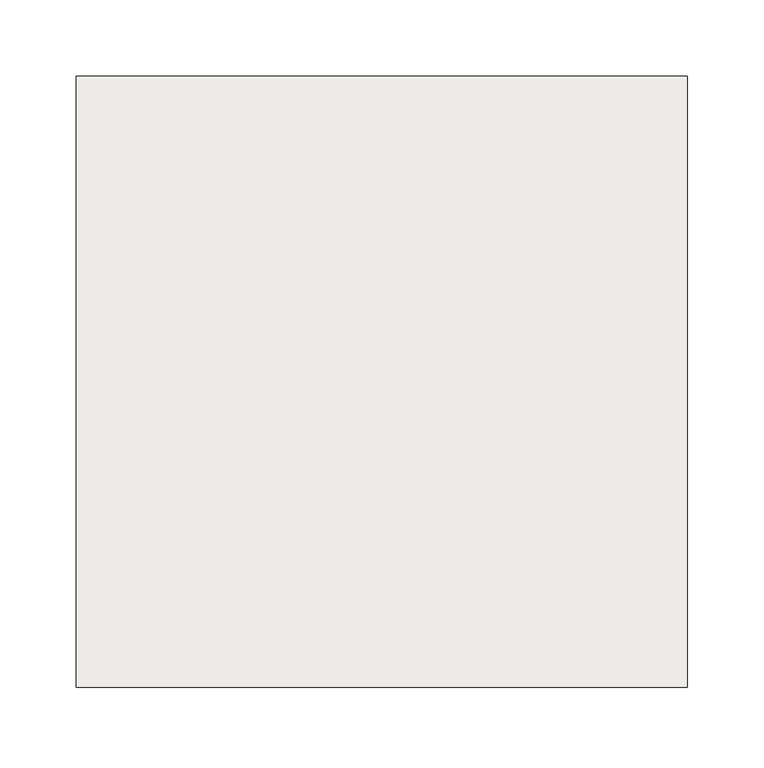
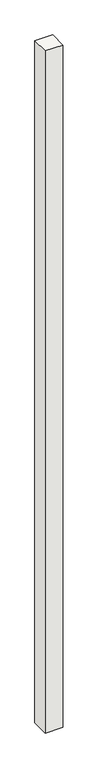
"""IFC4 building model written with IfcOpenShell, lengths in millimetres: footing geometry, NLRS_17_SFO_TLB_funderingspaal geheid beton prefab-AV-MMBPC_gen_rsf : heipaal beton prefab_gen__bxh 400x400."""

import ifcopenshell
import ifcopenshell.guid

model = None  # the IFC model being written
_history = None  # IfcOwnerHistory: only IFC2X3 demands one
_inside = {}  # id of a spatial element -> (the spatial element, [elements in it])
_under = {}  # id of a project, library or spatial element -> (it, [spatial elements below it])
_declared = {}  # id of a project -> (the project, [libraries it declares])
_typed = {}  # id of a type object -> (the type object, [elements of that type])
_made_of = {}  # id of a material, layer set ... -> (it, [elements and type objects made of it])


def new_model(schema):
    """Start an empty IFC model of exactly this schema.

    Asked for "IFC4X3", IfcOpenShell would pick the latest addendum, in which some entities
    have other attributes; the version numbers below select the first issue.
    IFC2X3 requires an IfcOwnerHistory on every rooted entity: one is made here for all.
    """
    global model, _history
    if schema == "IFC4X3":
        model = ifcopenshell.file(schema_version=(4, 3, 0, 0))
    else:
        model = ifcopenshell.file(schema=schema)
    _inside.clear()
    _under.clear()
    _declared.clear()
    _typed.clear()
    _made_of.clear()
    _history = None
    if model.schema == "IFC2X3":
        org = make("IfcOrganization", Name="unknown")
        user = make(
            "IfcPersonAndOrganization",
            ThePerson=make("IfcPerson", FamilyName="unknown"),
            TheOrganization=org,
        )
        app = make(
            "IfcApplication",
            ApplicationDeveloper=org,
            Version="unknown",
            ApplicationFullName="unknown",
            ApplicationIdentifier="unknown",
        )
        _history = make(
            "IfcOwnerHistory",
            OwningUser=user,
            OwningApplication=app,
            ChangeAction="ADDED",
            CreationDate=0,
        )
    return model


def make(cls, **values):
    """One entity of the class cls with the attributes given. An attribute that is None is left unset."""
    return model.create_entity(
        cls, **{name: value for name, value in values.items() if value is not None}
    )


def rooted(cls, **values):
    """An entity with a GlobalId (a new one), such as an element, a storey or a relation."""
    return make(cls, GlobalId=ifcopenshell.guid.new(), OwnerHistory=_history, **values)


def si_unit(unit_type, name, prefix=None):
    """IfcSIUnit, for example si_unit("LENGTHUNIT", "METRE", prefix="MILLI")."""
    return make("IfcSIUnit", UnitType=unit_type, Prefix=prefix, Name=name)


def assignment(units):
    """IfcUnitAssignment: the units of a project."""
    return None if units is None else make("IfcUnitAssignment", Units=units)


def point(xyz):
    """IfcCartesianPoint."""
    return None if xyz is None else make("IfcCartesianPoint", Coordinates=xyz)


def direction(xyz):
    """IfcDirection."""
    return None if xyz is None else make("IfcDirection", DirectionRatios=xyz)


def frame(location, z_axis=None, x_axis=None):
    """IfcAxis2Placement3D, a coordinate frame: its origin and axes. An axis left out is left unset."""
    return make(
        "IfcAxis2Placement3D",
        Location=point(location),
        Axis=direction(z_axis),
        RefDirection=direction(x_axis),
    )


def origin():
    """The frame at (0, 0, 0) with its axes left unset."""
    return frame((0.0, 0.0, 0.0))


def place(relative_to, where):
    """IfcLocalPlacement: puts the frame where relative to a parent placement (None: the world)."""
    return make(
        "IfcLocalPlacement", PlacementRelTo=relative_to, RelativePlacement=where
    )


def context(
    kind, dimensions, precision=None, world=None, true_north=None, identifier=None
):
    """IfcGeometricRepresentationContext, for example the 3D "Model" context."""
    return make(
        "IfcGeometricRepresentationContext",
        ContextIdentifier=identifier,
        ContextType=kind,
        CoordinateSpaceDimension=dimensions,
        Precision=precision,
        WorldCoordinateSystem=world,
        TrueNorth=true_north,
    )


def project(units=None, contexts=None):
    """IfcProject with its units and contexts."""
    return rooted(
        "IfcProject",
        Name="project",
        RepresentationContexts=contexts,
        UnitsInContext=assignment(units),
    )


def spatial(cls, under=None, at=None, **own):
    """A site, building, storey or space (cls), placed at a placement, below another one or the project."""
    s = rooted(cls, ObjectPlacement=at, **own)
    if under is not None:
        _under.setdefault(under.id(), (under, []))[1].append(s)
    return s


def polyline(points):
    """IfcPolyline through the points."""
    return make("IfcPolyline", Points=[point(p) for p in points])


def outline(outer, holes=None, kind="AREA"):
    """IfcArbitraryClosedProfileDef: a profile drawn as a closed curve; with holes, ...WithVoids."""
    if holes is None:
        return make("IfcArbitraryClosedProfileDef", ProfileType=kind, OuterCurve=outer)
    return make(
        "IfcArbitraryProfileDefWithVoids",
        ProfileType=kind,
        OuterCurve=outer,
        InnerCurves=holes,
    )


def extrude(swept, where, along, depth):
    """IfcExtrudedAreaSolid: the profile swept, set in the frame where, extruded along a direction by depth."""
    return make(
        "IfcExtrudedAreaSolid",
        SweptArea=swept,
        Position=where,
        ExtrudedDirection=direction(along),
        Depth=depth,
    )


def shape(context_of_items, identifier, shape_type, items):
    """IfcShapeRepresentation: the items that make up one representation, for example the "Body"."""
    return make(
        "IfcShapeRepresentation",
        ContextOfItems=context_of_items,
        RepresentationIdentifier=identifier,
        RepresentationType=shape_type,
        Items=items,
    )


def source(mapping_origin, context_of_items, identifier, shape_type, items):
    """IfcRepresentationMap: a shape defined once, which mapped items show again and again."""
    return make(
        "IfcRepresentationMap",
        MappingOrigin=mapping_origin,
        MappedRepresentation=shape(context_of_items, identifier, shape_type, items),
    )


def transform(
    local_origin,
    x_axis=None,
    y_axis=None,
    z_axis=None,
    scale=None,
    scale2=None,
    scale3=None,
    uniform=True,
):
    """IfcCartesianTransformationOperator3D, or its non-uniform kind. x_axis, y_axis, z_axis: its Axis1, 2, 3."""
    if uniform:
        return make(
            "IfcCartesianTransformationOperator3D",
            Axis1=direction(x_axis),
            Axis2=direction(y_axis),
            LocalOrigin=point(local_origin),
            Scale=scale,
            Axis3=direction(z_axis),
        )
    return make(
        "IfcCartesianTransformationOperator3DnonUniform",
        Axis1=direction(x_axis),
        Axis2=direction(y_axis),
        LocalOrigin=point(local_origin),
        Scale=scale,
        Axis3=direction(z_axis),
        Scale2=scale2,
        Scale3=scale3,
    )


def mapped(mapping_source, mapping_target):
    """IfcMappedItem: shows the shape of a source again, moved by a transform."""
    return make(
        "IfcMappedItem", MappingSource=mapping_source, MappingTarget=mapping_target
    )


def made_of(thing, what):
    """Note that an element or type object is made of a material, layer set ...; save() writes the relation."""
    if what is not None:
        _made_of.setdefault(what.id(), (what, []))[1].append(thing)
    return thing


def element(
    cls,
    number,
    at=None,
    inside=None,
    cuts=None,
    type_object=None,
    material=None,
    context=None,
    identifier="Body",
    shape_type=None,
    held_by="IfcProductDefinitionShape",
    body=None,
    shapes=None,
    **own,
):
    """One element of the class cls, such as IfcWall. Its Tag is "e" and its number.

    at: its placement. inside: the storey or other place that contains it. cuts: it is an
    opening in that element (IfcRelVoidsElement). A single representation is given by context,
    identifier, shape_type and body (its items); several are given by shapes. held_by: the class
    of the entity that holds the representations. save() writes the other relations.
    """
    e = rooted(cls, Tag="e%d" % number, ObjectPlacement=at, **own)
    if body is not None:
        shapes = [shape(context, identifier, shape_type, body)]
    if shapes is not None:
        e.Representation = make(held_by, Representations=shapes)
    if inside is not None:
        _inside.setdefault(inside.id(), (inside, []))[1].append(e)
    if cuts is not None:
        rooted(
            "IfcRelVoidsElement", RelatingBuildingElement=cuts, RelatedOpeningElement=e
        )
    if type_object is not None:
        _typed.setdefault(type_object.id(), (type_object, []))[1].append(e)
    return made_of(e, material)


def aggregate(whole, parts):
    """IfcRelAggregates: a whole, such as a stair, and the parts it consists of."""
    return rooted("IfcRelAggregates", RelatingObject=whole, RelatedObjects=parts)


def save(model, path):
    """Write the relations noted so far, then the file.

    IfcRelAggregates (storeys below a building ...), IfcRelContainedInSpatialStructure (elements
    in a storey), IfcRelDefinesByType, IfcRelAssociatesMaterial and IfcRelDeclares: one each for
    every whole, place, type object, material and project.
    """
    for whole, parts in _under.values():
        aggregate(whole, parts)
    for where, things in _inside.values():
        rooted(
            "IfcRelContainedInSpatialStructure",
            RelatedElements=things,
            RelatingStructure=where,
        )
    for kind, things in _typed.values():
        rooted("IfcRelDefinesByType", RelatedObjects=things, RelatingType=kind)
    for what, things in _made_of.values():
        rooted("IfcRelAssociatesMaterial", RelatedObjects=things, RelatingMaterial=what)
    for by, libraries in _declared.values():
        rooted("IfcRelDeclares", RelatingContext=by, RelatedDefinitions=libraries)
    model.write(path)


def footing_98706cf3(model_context):
    return source(origin(), model_context, "Body", "SweptSolid", [
        extrude(outline(polyline([(200.0, -200.0), (-200.0, -200.0), (-200.0, 200.0), (200.0, 200.0), (200.0, -200.0)])), frame((0.0, 0.0, -20000.0), z_axis=(0.0, 0.0, 1.0), x_axis=(1.0, 0.0, 0.0)), (0.0, 0.0, 1.0), 16280.0),
    ])


if __name__ == "__main__":
    model = new_model("IFC4")
    model_context = context("Model", 3, world=origin())
    ifc_project = project(units=[si_unit("LENGTHUNIT", "METRE", prefix="MILLI")], contexts=[model_context])
    site = spatial("IfcSite", under=ifc_project)
    building = spatial("IfcBuilding", under=site)
    placement = place(None, origin())
    footing_shape = footing_98706cf3(model_context)
    element("IfcFooting", 1, ObjectType="NLRS_17_SFO_TLB_funderingspaal geheid beton prefab-AV-MMBPC_gen_rsf : heipaal beton prefab_gen__bxh 400x400", at=placement, inside=building, context=model_context, shape_type="MappedRepresentation", body=[
        mapped(footing_shape, transform((0.0, 0.0, 0.0), x_axis=(1.0, 0.0, 0.0), y_axis=(0.0, 1.0, 0.0), z_axis=(0.0, 0.0, 1.0))),
    ])
    save(model, "model.ifc")

# Revit data of these elements
# Type "NLRS_17_SFO_TLB_funderingspaal geheid beton prefab-AV-MMBPC_gen_rsf : heipaal beton prefab_gen__bxh 400x400"
#   IfcExportAs = "IfcPile"
#   Type Comments = "prefab heipaal 400x400"
#   Model = " "
#   Manufacturer = " "
#   Description = "prefab heipaal 400x400"
#   Assembly Code = "17.21"
#   Width = 400 mm
#   Slanted Angle [instance default] = 0.00°
#   NLRS_S_draagvermogen_trek [instance default] = 0.00 kN
#   NLRS_S_draagvermogen_druk [instance default] = 0.00 kN
#   NLRS_C_lengte [instance default] = 1660 mm
#   NLRS_C_hoogte = 400 mm
#   NLRS_C_breedte = 400 mm
#   Height [instance default] = 1660 mm
#   Length [instance default] = 1660 mm
#   Angle [instance default] = 0.00°
#   Slanted [instance default] = 0
#   Structural Material = NLRS_f2_beton prefab_gen_rsf
#   Keynote = ""
# Element 1 (IfcFooting, "NLRS_17_SFO_TLB_funderingspaal geheid beton prefab-AV-MMBPC_gen_rsf : heipaal beton prefab_gen__bxh 400x400")
#   NLRS_C_lengte = 16280 mm
#   Height = 16280 mm
#   Length = 16280 mm
#   Materials on its faces: "NLRS_f2_beton prefab_gen_rsf"
# Materials
#   "NLRS_f2_beton prefab_gen_rsf": class "F - Niet gebakken kunststeen", colour RGB 129 133 118, transparency 0, Keynote = "f2", Manufacturer = "Revit Standards Foundation", URL = "www.revitstandards.org", Description = "beton prefab", Cost = 0
